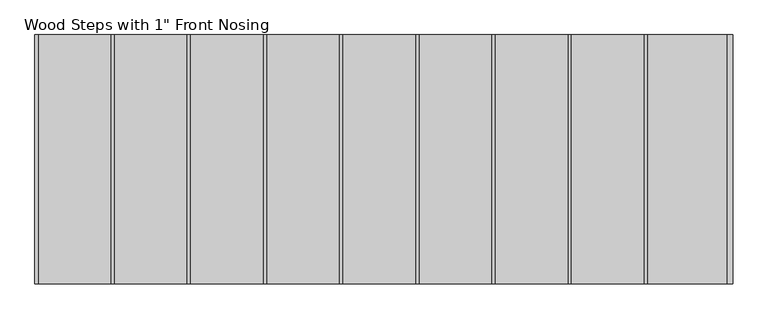
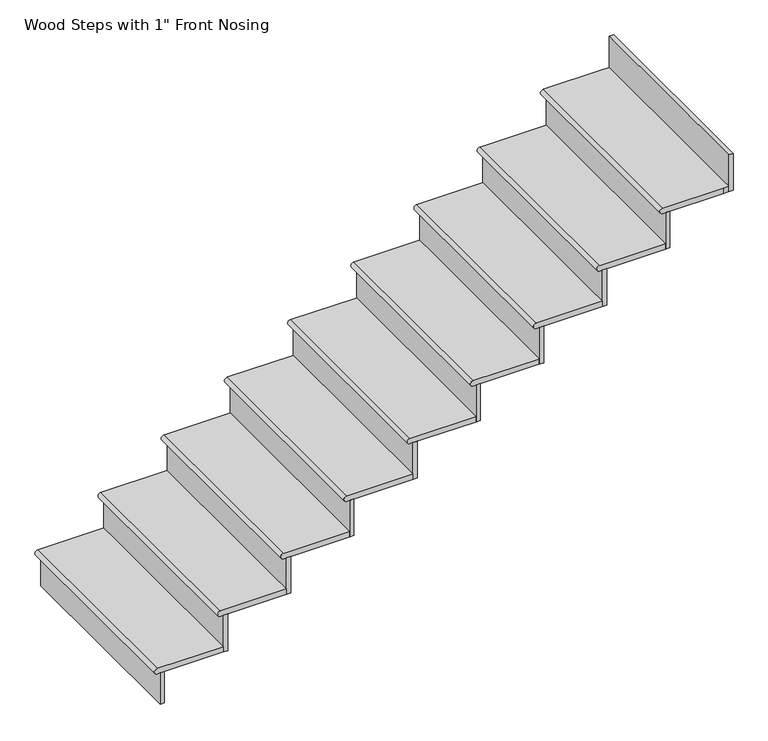
"""IFC4 building model written with IfcOpenShell, lengths in millimetres: stair flight geometry."""

import ifcopenshell
import ifcopenshell.guid

model = None  # the IFC model being written
_history = None  # IfcOwnerHistory: only IFC2X3 demands one
_inside = {}  # id of a spatial element -> (the spatial element, [elements in it])
_under = {}  # id of a project, library or spatial element -> (it, [spatial elements below it])
_declared = {}  # id of a project -> (the project, [libraries it declares])
_typed = {}  # id of a type object -> (the type object, [elements of that type])
_made_of = {}  # id of a material, layer set ... -> (it, [elements and type objects made of it])


def new_model(schema):
    """Start an empty IFC model of exactly this schema.

    Asked for "IFC4X3", IfcOpenShell would pick the latest addendum, in which some entities
    have other attributes; the version numbers below select the first issue.
    IFC2X3 requires an IfcOwnerHistory on every rooted entity: one is made here for all.
    """
    global model, _history
    if schema == "IFC4X3":
        model = ifcopenshell.file(schema_version=(4, 3, 0, 0))
    else:
        model = ifcopenshell.file(schema=schema)
    _inside.clear()
    _under.clear()
    _declared.clear()
    _typed.clear()
    _made_of.clear()
    _history = None
    if model.schema == "IFC2X3":
        org = make("IfcOrganization", Name="unknown")
        user = make(
            "IfcPersonAndOrganization",
            ThePerson=make("IfcPerson", FamilyName="unknown"),
            TheOrganization=org,
        )
        app = make(
            "IfcApplication",
            ApplicationDeveloper=org,
            Version="unknown",
            ApplicationFullName="unknown",
            ApplicationIdentifier="unknown",
        )
        _history = make(
            "IfcOwnerHistory",
            OwningUser=user,
            OwningApplication=app,
            ChangeAction="ADDED",
            CreationDate=0,
        )
    return model


def make(cls, **values):
    """One entity of the class cls with the attributes given. An attribute that is None is left unset."""
    return model.create_entity(
        cls, **{name: value for name, value in values.items() if value is not None}
    )


def rooted(cls, **values):
    """An entity with a GlobalId (a new one), such as an element, a storey or a relation."""
    return make(cls, GlobalId=ifcopenshell.guid.new(), OwnerHistory=_history, **values)


def si_unit(unit_type, name, prefix=None):
    """IfcSIUnit, for example si_unit("LENGTHUNIT", "METRE", prefix="MILLI")."""
    return make("IfcSIUnit", UnitType=unit_type, Prefix=prefix, Name=name)


def assignment(units):
    """IfcUnitAssignment: the units of a project."""
    return None if units is None else make("IfcUnitAssignment", Units=units)


def point(xyz):
    """IfcCartesianPoint."""
    return None if xyz is None else make("IfcCartesianPoint", Coordinates=xyz)


def direction(xyz):
    """IfcDirection."""
    return None if xyz is None else make("IfcDirection", DirectionRatios=xyz)


def frame(location, z_axis=None, x_axis=None):
    """IfcAxis2Placement3D, a coordinate frame: its origin and axes. An axis left out is left unset."""
    return make(
        "IfcAxis2Placement3D",
        Location=point(location),
        Axis=direction(z_axis),
        RefDirection=direction(x_axis),
    )


def origin():
    """The frame at (0, 0, 0) with its axes left unset."""
    return frame((0.0, 0.0, 0.0))


def place(relative_to, where):
    """IfcLocalPlacement: puts the frame where relative to a parent placement (None: the world)."""
    return make(
        "IfcLocalPlacement", PlacementRelTo=relative_to, RelativePlacement=where
    )


def context(
    kind, dimensions, precision=None, world=None, true_north=None, identifier=None
):
    """IfcGeometricRepresentationContext, for example the 3D "Model" context."""
    return make(
        "IfcGeometricRepresentationContext",
        ContextIdentifier=identifier,
        ContextType=kind,
        CoordinateSpaceDimension=dimensions,
        Precision=precision,
        WorldCoordinateSystem=world,
        TrueNorth=true_north,
    )


def project(units=None, contexts=None):
    """IfcProject with its units and contexts."""
    return rooted(
        "IfcProject",
        Name="project",
        RepresentationContexts=contexts,
        UnitsInContext=assignment(units),
    )


def spatial(cls, under=None, at=None, **own):
    """A site, building, storey or space (cls), placed at a placement, below another one or the project."""
    s = rooted(cls, ObjectPlacement=at, **own)
    if under is not None:
        _under.setdefault(under.id(), (under, []))[1].append(s)
    return s


def circle_curve(where, radius):
    """IfcCircle in the frame where."""
    return make("IfcCircle", Position=where, Radius=radius)


def faces_of(points, faces, orient=None, outer=None):
    """IfcFace entities. A face is a list of loops; a loop is a list of indices into points, from 0.

    orient and outer hold one flag for each loop. By default every Orientation is true, the
    first loop of a face is its IfcFaceOuterBound and the others are IfcFaceBound.
    """
    made = []
    for i, loops in enumerate(faces):
        bounds = []
        for j, loop in enumerate(loops):
            is_outer = j == 0 if outer is None else outer[i][j]
            bounds.append(
                make(
                    "IfcFaceOuterBound" if is_outer else "IfcFaceBound",
                    Bound=make("IfcPolyLoop", Polygon=[points[k] for k in loop]),
                    Orientation=True if orient is None else orient[i][j],
                )
            )
        made.append(make("IfcFace", Bounds=bounds))
    return made


def faceted_brep(points, faces, orient=None, outer=None, voids=None):
    """IfcFacetedBrep: a solid bounded by flat faces; with voids (closed shells), ...WithVoids."""
    shared = [point(p) for p in points]
    hull = make("IfcClosedShell", CfsFaces=faces_of(shared, faces, orient, outer))
    if voids is None:
        return make("IfcFacetedBrep", Outer=hull)
    return make(
        "IfcFacetedBrepWithVoids",
        Outer=hull,
        Voids=[
            make(cls, CfsFaces=faces_of(shared, fs, o, b)) for cls, fs, o, b in voids
        ],
    )


def shape(context_of_items, identifier, shape_type, items):
    """IfcShapeRepresentation: the items that make up one representation, for example the "Body"."""
    return make(
        "IfcShapeRepresentation",
        ContextOfItems=context_of_items,
        RepresentationIdentifier=identifier,
        RepresentationType=shape_type,
        Items=items,
    )


def source(mapping_origin, context_of_items, identifier, shape_type, items):
    """IfcRepresentationMap: a shape defined once, which mapped items show again and again."""
    return make(
        "IfcRepresentationMap",
        MappingOrigin=mapping_origin,
        MappedRepresentation=shape(context_of_items, identifier, shape_type, items),
    )


def transform(
    local_origin,
    x_axis=None,
    y_axis=None,
    z_axis=None,
    scale=None,
    scale2=None,
    scale3=None,
    uniform=True,
):
    """IfcCartesianTransformationOperator3D, or its non-uniform kind. x_axis, y_axis, z_axis: its Axis1, 2, 3."""
    if uniform:
        return make(
            "IfcCartesianTransformationOperator3D",
            Axis1=direction(x_axis),
            Axis2=direction(y_axis),
            LocalOrigin=point(local_origin),
            Scale=scale,
            Axis3=direction(z_axis),
        )
    return make(
        "IfcCartesianTransformationOperator3DnonUniform",
        Axis1=direction(x_axis),
        Axis2=direction(y_axis),
        LocalOrigin=point(local_origin),
        Scale=scale,
        Axis3=direction(z_axis),
        Scale2=scale2,
        Scale3=scale3,
    )


def mapped(mapping_source, mapping_target):
    """IfcMappedItem: shows the shape of a source again, moved by a transform."""
    return make(
        "IfcMappedItem", MappingSource=mapping_source, MappingTarget=mapping_target
    )


def made_of(thing, what):
    """Note that an element or type object is made of a material, layer set ...; save() writes the relation."""
    if what is not None:
        _made_of.setdefault(what.id(), (what, []))[1].append(thing)
    return thing


def element(
    cls,
    number,
    at=None,
    inside=None,
    cuts=None,
    type_object=None,
    material=None,
    context=None,
    identifier="Body",
    shape_type=None,
    held_by="IfcProductDefinitionShape",
    body=None,
    shapes=None,
    **own,
):
    """One element of the class cls, such as IfcWall. Its Tag is "e" and its number.

    at: its placement. inside: the storey or other place that contains it. cuts: it is an
    opening in that element (IfcRelVoidsElement). A single representation is given by context,
    identifier, shape_type and body (its items); several are given by shapes. held_by: the class
    of the entity that holds the representations. save() writes the other relations.
    """
    e = rooted(cls, Tag="e%d" % number, ObjectPlacement=at, **own)
    if body is not None:
        shapes = [shape(context, identifier, shape_type, body)]
    if shapes is not None:
        e.Representation = make(held_by, Representations=shapes)
    if inside is not None:
        _inside.setdefault(inside.id(), (inside, []))[1].append(e)
    if cuts is not None:
        rooted(
            "IfcRelVoidsElement", RelatingBuildingElement=cuts, RelatedOpeningElement=e
        )
    if type_object is not None:
        _typed.setdefault(type_object.id(), (type_object, []))[1].append(e)
    return made_of(e, material)


def aggregate(whole, parts):
    """IfcRelAggregates: a whole, such as a stair, and the parts it consists of."""
    return rooted("IfcRelAggregates", RelatingObject=whole, RelatedObjects=parts)


def save(model, path):
    """Write the relations noted so far, then the file.

    IfcRelAggregates (storeys below a building ...), IfcRelContainedInSpatialStructure (elements
    in a storey), IfcRelDefinesByType, IfcRelAssociatesMaterial and IfcRelDeclares: one each for
    every whole, place, type object, material and project.
    """
    for whole, parts in _under.values():
        aggregate(whole, parts)
    for where, things in _inside.values():
        rooted(
            "IfcRelContainedInSpatialStructure",
            RelatedElements=things,
            RelatingStructure=where,
        )
    for kind, things in _typed.values():
        rooted("IfcRelDefinesByType", RelatedObjects=things, RelatingType=kind)
    for what, things in _made_of.values():
        rooted("IfcRelAssociatesMaterial", RelatedObjects=things, RelatingMaterial=what)
    for by, libraries in _declared.values():
        rooted("IfcRelDeclares", RelatingContext=by, RelatedDefinitions=libraries)
    model.write(path)


def plane_surface(at):
    """IfcPlane: the flat surface through the origin of the frame at, square to its z axis."""
    return make("IfcPlane", Position=at)


def cylinder_surface(at, radius):
    """IfcCylindricalSurface: all points at the distance radius from the z axis of the frame at."""
    return make("IfcCylindricalSurface", Position=at, Radius=radius)


def advanced_brep(points, edges, surfaces, faces):
    """IfcAdvancedBrep: a solid bounded by faces that lie on surfaces and meet in shared edges.

    An edge is (start, end): straight between two places in points (the first is 0);
    or (start, end, curve); or (start, end, curve, False) where it runs against its curve.
    A face is (place in surfaces, loops), or (place, loops, False) where it looks against
    its surface's normal. A loop lists edges by number (the first is 1), with a minus sign
    where the edge is run from its end to its start. The first loop is the outer one.
    """
    corners = [point(p) for p in points]
    vertices = [make("IfcVertexPoint", VertexGeometry=c) for c in corners]
    made = []
    for start, end, *more in edges:
        made.append(
            make(
                "IfcEdgeCurve",
                EdgeStart=vertices[start],
                EdgeEnd=vertices[end],
                EdgeGeometry=more[0] if more else make("IfcPolyline", Points=[corners[start], corners[end]]),
                SameSense=more[1] if len(more) > 1 else True,
            )
        )
    hull = []
    for where, loops, *sense in faces:
        bounds = []
        for j, loop in enumerate(loops):
            ring = [make("IfcOrientedEdge", EdgeElement=made[abs(k) - 1], Orientation=k > 0) for k in loop]
            bounds.append(
                make(
                    "IfcFaceOuterBound" if j == 0 else "IfcFaceBound",
                    Bound=make("IfcEdgeLoop", EdgeList=ring),
                    Orientation=True,
                )
            )
        hull.append(make("IfcAdvancedFace", Bounds=bounds, FaceSurface=surfaces[where], SameSense=sense[0] if sense else True))
    return make("IfcAdvancedBrep", Outer=make("IfcClosedShell", CfsFaces=hull))


def stair_flight_bb49cb81(model_context):
    return source(origin(), model_context, "Body", "SolidModel", [
        advanced_brep(
        [(3725.1741968, -13363.3557429, 146.05), (3725.1741968, -13363.3557429, 171.45), (3725.1741968, -12448.9557429, 171.45), (3725.1741968, -12448.9557429, 146.05), (4017.2741968, -12448.9557429, 171.45), (4017.2741968, -13363.3557429, 171.45), (4017.2741968, -12448.9557429, 146.05), (4017.2741968, -13363.3557429, 146.05)],
        [
            (0, 1, circle_curve(frame((3725.1741968, -13363.3557429, 158.75), z_axis=(0.0, 1.0, 0.0), x_axis=(1.0, 0.0, 0.0)), 12.7)),
            (1, 2),
            (2, 3, circle_curve(frame((3725.1741968, -12448.9557429, 158.75), z_axis=(0.0, -1.0, 0.0), x_axis=(1.0, 0.0, 0.0)), 12.7)),
            (3, 0),
            (4, 2),
            (1, 5),
            (5, 4),
            (3, 6),
            (6, 7),
            (7, 0),
            (4, 6),
            (7, 5),
        ],
        [
            cylinder_surface(frame((3725.1741968, -13363.3557429, 158.75), z_axis=(0.0, -1.0, 0.0), x_axis=(1.0, 0.0, 0.0)), 12.7),
            plane_surface(frame((3712.4741968, -12448.9557429, 171.45), z_axis=(0.0, 0.0, 1.0), x_axis=(-1.0, 0.0, 0.0))),
            plane_surface(frame((3712.4741968, -12448.9557429, 146.05), z_axis=(0.0, 0.0, -1.0), x_axis=(1.0, 0.0, 0.0))),
            plane_surface(frame((4017.2741968, -12448.9557429, 171.45), z_axis=(0.0, 1.0, 0.0), x_axis=(0.0, 0.0, -1.0))),
            plane_surface(frame((3725.1741968, -13363.3557429, 171.45), z_axis=(0.0, -1.0, 0.0), x_axis=(0.0, 0.0, -1.0))),
            plane_surface(frame((4017.2741968, -13363.3557429, 171.45), z_axis=(1.0, 0.0, 0.0), x_axis=(0.0, 0.0, -1.0))),
        ],
        [
            (0, [[1, 2, 3, 4]]),
            (1, [[5, -2, 6, 7]]),
            (2, [[8, 9, 10, -4]]),
            (3, [[-5, 11, -8, -3]]),
            (4, [[-6, -1, -10, 12]]),
            (5, [[-7, -12, -9, -11]]),
        ],
    ),
        faceted_brep([(3737.8741968, -13363.3557429, 146.05), (3737.8741968, -13363.3557429, 0.0), (3756.9241968, -13363.3557429, 0.0), (3756.9241968, -13363.3557429, 146.05), (3737.8741968, -12448.9557429, 146.05), (3756.9241968, -12448.9557429, 146.05), (3756.9241968, -12448.9557429, 0.0), (3737.8741968, -12448.9557429, 0.0)], [[[0, 1, 2, 3]], [[4, 5, 6, 7]], [[1, 0, 4, 7]], [[2, 1, 7, 6]], [[3, 2, 6, 5]], [[0, 3, 5, 4]]]),
        faceted_brep([(4017.2741968, -13363.3557429, 317.5), (4017.2741968, -13363.3557429, 146.05), (4036.3241968, -13363.3557429, 146.05), (4036.3241968, -13363.3557429, 317.5), (4017.2741968, -12448.9557429, 317.5), (4036.3241968, -12448.9557429, 317.5), (4036.3241968, -12448.9557429, 146.05), (4017.2741968, -12448.9557429, 146.05)], [[[0, 1, 2, 3]], [[4, 5, 6, 7]], [[1, 0, 4, 7]], [[2, 1, 7, 6]], [[3, 2, 6, 5]], [[0, 3, 5, 4]]]),
        advanced_brep(
        [(4296.6741968, -12448.9557429, 342.9), (4004.5741968, -12448.9557429, 342.9), (4004.5741968, -13363.3557429, 342.9), (4296.6741968, -13363.3557429, 342.9), (4004.5741968, -12448.9557429, 317.5), (4296.6741968, -12448.9557429, 317.5), (4296.6741968, -13363.3557429, 317.5), (4004.5741968, -13363.3557429, 317.5)],
        [
            (0, 1),
            (1, 2),
            (2, 3),
            (3, 0),
            (4, 5),
            (5, 6),
            (6, 7),
            (7, 4),
            (0, 5),
            (4, 1, circle_curve(frame((4004.5741968, -12448.9557429, 330.2), z_axis=(0.0, 1.0, 0.0), x_axis=(1.0, 0.0, 0.0)), 12.7)),
            (2, 7, circle_curve(frame((4004.5741968, -13363.3557429, 330.2), z_axis=(0.0, -1.0, 0.0), x_axis=(1.0, 0.0, 0.0)), 12.7)),
            (6, 3),
        ],
        [
            plane_surface(frame((3712.4741968, -12448.9557429, 342.9), z_axis=(0.0, 0.0, 1.0), x_axis=(-1.0, 0.0, 0.0))),
            plane_surface(frame((3712.4741968, -12448.9557429, 317.5), z_axis=(0.0, 0.0, -1.0), x_axis=(1.0, 0.0, 0.0))),
            plane_surface(frame((4296.6741968, -12448.9557429, 342.9), z_axis=(0.0, 1.0, 0.0), x_axis=(0.0, 0.0, -1.0))),
            plane_surface(frame((4004.5741968, -13363.3557429, 342.9), z_axis=(0.0, -1.0, 0.0), x_axis=(0.0, 0.0, -1.0))),
            plane_surface(frame((4296.6741968, -13363.3557429, 342.9), z_axis=(1.0, 0.0, 0.0), x_axis=(0.0, 0.0, -1.0))),
            cylinder_surface(frame((4004.5741968, -13363.3557429, 330.2), z_axis=(0.0, -1.0, 0.0), x_axis=(1.0, 0.0, 0.0)), 12.7),
        ],
        [
            (0, [[1, 2, 3, 4]]),
            (1, [[5, 6, 7, 8]]),
            (2, [[-1, 9, -5, 10]]),
            (3, [[-3, 11, -7, 12]]),
            (4, [[-4, -12, -6, -9]]),
            (5, [[-11, -2, -10, -8]]),
        ],
    ),
        faceted_brep([(4296.6741968, -13363.3557429, 488.95), (4296.6741968, -13363.3557429, 317.5), (4315.7241968, -13363.3557429, 317.5), (4315.7241968, -13363.3557429, 488.95), (4296.6741968, -12448.9557429, 488.95), (4315.7241968, -12448.9557429, 488.95), (4315.7241968, -12448.9557429, 317.5), (4296.6741968, -12448.9557429, 317.5)], [[[0, 1, 2, 3]], [[4, 5, 6, 7]], [[1, 0, 4, 7]], [[2, 1, 7, 6]], [[3, 2, 6, 5]], [[0, 3, 5, 4]]]),
        advanced_brep(
        [(4576.0741968, -12448.9557429, 514.35), (4283.9741968, -12448.9557429, 514.35), (4283.9741968, -13363.3557429, 514.35), (4576.0741968, -13363.3557429, 514.35), (4283.9741968, -12448.9557429, 488.95), (4576.0741968, -12448.9557429, 488.95), (4576.0741968, -13363.3557429, 488.95), (4283.9741968, -13363.3557429, 488.95)],
        [
            (0, 1),
            (1, 2),
            (2, 3),
            (3, 0),
            (4, 5),
            (5, 6),
            (6, 7),
            (7, 4),
            (0, 5),
            (4, 1, circle_curve(frame((4283.9741968, -12448.9557429, 501.65), z_axis=(0.0, 1.0, 0.0), x_axis=(1.0, 0.0, 0.0)), 12.7)),
            (2, 7, circle_curve(frame((4283.9741968, -13363.3557429, 501.65), z_axis=(0.0, -1.0, 0.0), x_axis=(1.0, 0.0, 0.0)), 12.7)),
            (6, 3),
        ],
        [
            plane_surface(frame((3991.8741968, -12448.9557429, 514.35), z_axis=(0.0, 0.0, 1.0), x_axis=(-1.0, 0.0, 0.0))),
            plane_surface(frame((3991.8741968, -12448.9557429, 488.95), z_axis=(0.0, 0.0, -1.0), x_axis=(1.0, 0.0, 0.0))),
            plane_surface(frame((4576.0741968, -12448.9557429, 514.35), z_axis=(0.0, 1.0, 0.0), x_axis=(0.0, 0.0, -1.0))),
            plane_surface(frame((4283.9741968, -13363.3557429, 514.35), z_axis=(0.0, -1.0, 0.0), x_axis=(0.0, 0.0, -1.0))),
            plane_surface(frame((4576.0741968, -13363.3557429, 514.35), z_axis=(1.0, 0.0, 0.0), x_axis=(0.0, 0.0, -1.0))),
            cylinder_surface(frame((4283.9741968, -13363.3557429, 501.65), z_axis=(0.0, -1.0, 0.0), x_axis=(1.0, 0.0, 0.0)), 12.7),
        ],
        [
            (0, [[1, 2, 3, 4]]),
            (1, [[5, 6, 7, 8]]),
            (2, [[-1, 9, -5, 10]]),
            (3, [[-3, 11, -7, 12]]),
            (4, [[-4, -12, -6, -9]]),
            (5, [[-11, -2, -10, -8]]),
        ],
    ),
        faceted_brep([(4576.0741968, -13363.3557429, 660.4), (4576.0741968, -13363.3557429, 488.95), (4595.1241968, -13363.3557429, 488.95), (4595.1241968, -13363.3557429, 660.4), (4576.0741968, -12448.9557429, 660.4), (4595.1241968, -12448.9557429, 660.4), (4595.1241968, -12448.9557429, 488.95), (4576.0741968, -12448.9557429, 488.95)], [[[0, 1, 2, 3]], [[4, 5, 6, 7]], [[1, 0, 4, 7]], [[2, 1, 7, 6]], [[3, 2, 6, 5]], [[0, 3, 5, 4]]]),
        advanced_brep(
        [(4855.4741968, -12448.9557429, 685.8), (4563.3741968, -12448.9557429, 685.8), (4563.3741968, -13363.3557429, 685.8), (4855.4741968, -13363.3557429, 685.8), (4563.3741968, -12448.9557429, 660.4), (4855.4741968, -12448.9557429, 660.4), (4855.4741968, -13363.3557429, 660.4), (4563.3741968, -13363.3557429, 660.4)],
        [
            (0, 1),
            (1, 2),
            (2, 3),
            (3, 0),
            (4, 5),
            (5, 6),
            (6, 7),
            (7, 4),
            (0, 5),
            (4, 1, circle_curve(frame((4563.3741968, -12448.9557429, 673.1), z_axis=(0.0, 1.0, 0.0), x_axis=(1.0, 0.0, 0.0)), 12.7)),
            (2, 7, circle_curve(frame((4563.3741968, -13363.3557429, 673.1), z_axis=(0.0, -1.0, 0.0), x_axis=(1.0, 0.0, 0.0)), 12.7)),
            (6, 3),
        ],
        [
            plane_surface(frame((4271.2741968, -12448.9557429, 685.8), z_axis=(0.0, 0.0, 1.0), x_axis=(-1.0, 0.0, 0.0))),
            plane_surface(frame((4271.2741968, -12448.9557429, 660.4), z_axis=(0.0, 0.0, -1.0), x_axis=(1.0, 0.0, 0.0))),
            plane_surface(frame((4855.4741968, -12448.9557429, 685.8), z_axis=(0.0, 1.0, 0.0), x_axis=(0.0, 0.0, -1.0))),
            plane_surface(frame((4563.3741968, -13363.3557429, 685.8), z_axis=(0.0, -1.0, 0.0), x_axis=(0.0, 0.0, -1.0))),
            plane_surface(frame((4855.4741968, -13363.3557429, 685.8), z_axis=(1.0, 0.0, 0.0), x_axis=(0.0, 0.0, -1.0))),
            cylinder_surface(frame((4563.3741968, -13363.3557429, 673.1), z_axis=(0.0, -1.0, 0.0), x_axis=(1.0, 0.0, 0.0)), 12.7),
        ],
        [
            (0, [[1, 2, 3, 4]]),
            (1, [[5, 6, 7, 8]]),
            (2, [[-1, 9, -5, 10]]),
            (3, [[-3, 11, -7, 12]]),
            (4, [[-4, -12, -6, -9]]),
            (5, [[-11, -2, -10, -8]]),
        ],
    ),
        faceted_brep([(4855.4741968, -13363.3557429, 831.85), (4855.4741968, -13363.3557429, 660.4), (4874.5241968, -13363.3557429, 660.4), (4874.5241968, -13363.3557429, 831.85), (4855.4741968, -12448.9557429, 831.85), (4874.5241968, -12448.9557429, 831.85), (4874.5241968, -12448.9557429, 660.4), (4855.4741968, -12448.9557429, 660.4)], [[[0, 1, 2, 3]], [[4, 5, 6, 7]], [[1, 0, 4, 7]], [[2, 1, 7, 6]], [[3, 2, 6, 5]], [[0, 3, 5, 4]]]),
        advanced_brep(
        [(5134.8741968, -12448.9557429, 857.25), (4842.7741968, -12448.9557429, 857.25), (4842.7741968, -13363.3557429, 857.25), (5134.8741968, -13363.3557429, 857.25), (4842.7741968, -12448.9557429, 831.85), (5134.8741968, -12448.9557429, 831.85), (5134.8741968, -13363.3557429, 831.85), (4842.7741968, -13363.3557429, 831.85)],
        [
            (0, 1),
            (1, 2),
            (2, 3),
            (3, 0),
            (4, 5),
            (5, 6),
            (6, 7),
            (7, 4),
            (0, 5),
            (4, 1, circle_curve(frame((4842.7741968, -12448.9557429, 844.55), z_axis=(0.0, 1.0, 0.0), x_axis=(1.0, 0.0, 0.0)), 12.7)),
            (2, 7, circle_curve(frame((4842.7741968, -13363.3557429, 844.55), z_axis=(0.0, -1.0, 0.0), x_axis=(1.0, 0.0, 0.0)), 12.7)),
            (6, 3),
        ],
        [
            plane_surface(frame((4550.6741968, -12448.9557429, 857.25), z_axis=(0.0, 0.0, 1.0), x_axis=(-1.0, 0.0, 0.0))),
            plane_surface(frame((4550.6741968, -12448.9557429, 831.85), z_axis=(0.0, 0.0, -1.0), x_axis=(1.0, 0.0, 0.0))),
            plane_surface(frame((5134.8741968, -12448.9557429, 857.25), z_axis=(0.0, 1.0, 0.0), x_axis=(0.0, 0.0, -1.0))),
            plane_surface(frame((4842.7741968, -13363.3557429, 857.25), z_axis=(0.0, -1.0, 0.0), x_axis=(0.0, 0.0, -1.0))),
            plane_surface(frame((5134.8741968, -13363.3557429, 857.25), z_axis=(1.0, 0.0, 0.0), x_axis=(0.0, 0.0, -1.0))),
            cylinder_surface(frame((4842.7741968, -13363.3557429, 844.55), z_axis=(0.0, -1.0, 0.0), x_axis=(1.0, 0.0, 0.0)), 12.7),
        ],
        [
            (0, [[1, 2, 3, 4]]),
            (1, [[5, 6, 7, 8]]),
            (2, [[-1, 9, -5, 10]]),
            (3, [[-3, 11, -7, 12]]),
            (4, [[-4, -12, -6, -9]]),
            (5, [[-11, -2, -10, -8]]),
        ],
    ),
        faceted_brep([(5134.8741968, -13363.3557429, 1003.3), (5134.8741968, -13363.3557429, 831.85), (5153.9241968, -13363.3557429, 831.85), (5153.9241968, -13363.3557429, 1003.3), (5134.8741968, -12448.9557429, 1003.3), (5153.9241968, -12448.9557429, 1003.3), (5153.9241968, -12448.9557429, 831.85), (5134.8741968, -12448.9557429, 831.85)], [[[0, 1, 2, 3]], [[4, 5, 6, 7]], [[1, 0, 4, 7]], [[2, 1, 7, 6]], [[3, 2, 6, 5]], [[0, 3, 5, 4]]]),
        advanced_brep(
        [(5414.2741968, -12448.9557429, 1028.7), (5122.1741968, -12448.9557429, 1028.7), (5122.1741968, -13363.3557429, 1028.7), (5414.2741968, -13363.3557429, 1028.7), (5122.1741968, -12448.9557429, 1003.3), (5414.2741968, -12448.9557429, 1003.3), (5414.2741968, -13363.3557429, 1003.3), (5122.1741968, -13363.3557429, 1003.3)],
        [
            (0, 1),
            (1, 2),
            (2, 3),
            (3, 0),
            (4, 5),
            (5, 6),
            (6, 7),
            (7, 4),
            (0, 5),
            (4, 1, circle_curve(frame((5122.1741968, -12448.9557429, 1016.0), z_axis=(0.0, 1.0, 0.0), x_axis=(1.0, 0.0, 0.0)), 12.7)),
            (2, 7, circle_curve(frame((5122.1741968, -13363.3557429, 1016.0), z_axis=(0.0, -1.0, 0.0), x_axis=(1.0, 0.0, 0.0)), 12.7)),
            (6, 3),
        ],
        [
            plane_surface(frame((4830.0741968, -12448.9557429, 1028.7), z_axis=(0.0, 0.0, 1.0), x_axis=(-1.0, 0.0, 0.0))),
            plane_surface(frame((4830.0741968, -12448.9557429, 1003.3), z_axis=(0.0, 0.0, -1.0), x_axis=(1.0, 0.0, 0.0))),
            plane_surface(frame((5414.2741968, -12448.9557429, 1028.7), z_axis=(0.0, 1.0, 0.0), x_axis=(0.0, 0.0, -1.0))),
            plane_surface(frame((5122.1741968, -13363.3557429, 1028.7), z_axis=(0.0, -1.0, 0.0), x_axis=(0.0, 0.0, -1.0))),
            plane_surface(frame((5414.2741968, -13363.3557429, 1028.7), z_axis=(1.0, 0.0, 0.0), x_axis=(0.0, 0.0, -1.0))),
            cylinder_surface(frame((5122.1741968, -13363.3557429, 1016.0), z_axis=(0.0, -1.0, 0.0), x_axis=(1.0, 0.0, 0.0)), 12.7),
        ],
        [
            (0, [[1, 2, 3, 4]]),
            (1, [[5, 6, 7, 8]]),
            (2, [[-1, 9, -5, 10]]),
            (3, [[-3, 11, -7, 12]]),
            (4, [[-4, -12, -6, -9]]),
            (5, [[-11, -2, -10, -8]]),
        ],
    ),
        faceted_brep([(5414.2741968, -13363.3557429, 1174.75), (5414.2741968, -13363.3557429, 1003.3), (5433.3241968, -13363.3557429, 1003.3), (5433.3241968, -13363.3557429, 1174.75), (5414.2741968, -12448.9557429, 1174.75), (5433.3241968, -12448.9557429, 1174.75), (5433.3241968, -12448.9557429, 1003.3), (5414.2741968, -12448.9557429, 1003.3)], [[[0, 1, 2, 3]], [[4, 5, 6, 7]], [[1, 0, 4, 7]], [[2, 1, 7, 6]], [[3, 2, 6, 5]], [[0, 3, 5, 4]]]),
        advanced_brep(
        [(5693.6741968, -12448.9557429, 1200.15), (5401.5741968, -12448.9557429, 1200.15), (5401.5741968, -13363.3557429, 1200.15), (5693.6741968, -13363.3557429, 1200.15), (5401.5741968, -12448.9557429, 1174.75), (5693.6741968, -12448.9557429, 1174.75), (5693.6741968, -13363.3557429, 1174.75), (5401.5741968, -13363.3557429, 1174.75)],
        [
            (0, 1),
            (1, 2),
            (2, 3),
            (3, 0),
            (4, 5),
            (5, 6),
            (6, 7),
            (7, 4),
            (0, 5),
            (4, 1, circle_curve(frame((5401.5741968, -12448.9557429, 1187.45), z_axis=(0.0, 1.0, 0.0), x_axis=(1.0, 0.0, 0.0)), 12.7)),
            (2, 7, circle_curve(frame((5401.5741968, -13363.3557429, 1187.45), z_axis=(0.0, -1.0, 0.0), x_axis=(1.0, 0.0, 0.0)), 12.7)),
            (6, 3),
        ],
        [
            plane_surface(frame((5109.4741968, -12448.9557429, 1200.15), z_axis=(0.0, 0.0, 1.0), x_axis=(-1.0, 0.0, 0.0))),
            plane_surface(frame((5109.4741968, -12448.9557429, 1174.75), z_axis=(0.0, 0.0, -1.0), x_axis=(1.0, 0.0, 0.0))),
            plane_surface(frame((5693.6741968, -12448.9557429, 1200.15), z_axis=(0.0, 1.0, 0.0), x_axis=(0.0, 0.0, -1.0))),
            plane_surface(frame((5401.5741968, -13363.3557429, 1200.15), z_axis=(0.0, -1.0, 0.0), x_axis=(0.0, 0.0, -1.0))),
            plane_surface(frame((5693.6741968, -13363.3557429, 1200.15), z_axis=(1.0, 0.0, 0.0), x_axis=(0.0, 0.0, -1.0))),
            cylinder_surface(frame((5401.5741968, -13363.3557429, 1187.45), z_axis=(0.0, -1.0, 0.0), x_axis=(1.0, 0.0, 0.0)), 12.7),
        ],
        [
            (0, [[1, 2, 3, 4]]),
            (1, [[5, 6, 7, 8]]),
            (2, [[-1, 9, -5, 10]]),
            (3, [[-3, 11, -7, 12]]),
            (4, [[-4, -12, -6, -9]]),
            (5, [[-11, -2, -10, -8]]),
        ],
    ),
        faceted_brep([(5693.6741968, -13363.3557429, 1346.2), (5693.6741968, -13363.3557429, 1174.75), (5712.7241968, -13363.3557429, 1174.75), (5712.7241968, -13363.3557429, 1346.2), (5693.6741968, -12448.9557429, 1346.2), (5712.7241968, -12448.9557429, 1346.2), (5712.7241968, -12448.9557429, 1174.75), (5693.6741968, -12448.9557429, 1174.75)], [[[0, 1, 2, 3]], [[4, 5, 6, 7]], [[1, 0, 4, 7]], [[2, 1, 7, 6]], [[3, 2, 6, 5]], [[0, 3, 5, 4]]]),
        advanced_brep(
        [(5973.0741968, -12448.9557429, 1371.6), (5680.9741968, -12448.9557429, 1371.6), (5680.9741968, -13363.3557429, 1371.6), (5973.0741968, -13363.3557429, 1371.6), (5680.9741968, -12448.9557429, 1346.2), (5973.0741968, -12448.9557429, 1346.2), (5973.0741968, -13363.3557429, 1346.2), (5680.9741968, -13363.3557429, 1346.2)],
        [
            (0, 1),
            (1, 2),
            (2, 3),
            (3, 0),
            (4, 5),
            (5, 6),
            (6, 7),
            (7, 4),
            (0, 5),
            (4, 1, circle_curve(frame((5680.9741968, -12448.9557429, 1358.9), z_axis=(0.0, 1.0, 0.0), x_axis=(1.0, 0.0, 0.0)), 12.7)),
            (2, 7, circle_curve(frame((5680.9741968, -13363.3557429, 1358.9), z_axis=(0.0, -1.0, 0.0), x_axis=(1.0, 0.0, 0.0)), 12.7)),
            (6, 3),
        ],
        [
            plane_surface(frame((5388.8741968, -12448.9557429, 1371.6), z_axis=(0.0, 0.0, 1.0), x_axis=(-1.0, 0.0, 0.0))),
            plane_surface(frame((5388.8741968, -12448.9557429, 1346.2), z_axis=(0.0, 0.0, -1.0), x_axis=(1.0, 0.0, 0.0))),
            plane_surface(frame((5973.0741968, -12448.9557429, 1371.6), z_axis=(0.0, 1.0, 0.0), x_axis=(0.0, 0.0, -1.0))),
            plane_surface(frame((5680.9741968, -13363.3557429, 1371.6), z_axis=(0.0, -1.0, 0.0), x_axis=(0.0, 0.0, -1.0))),
            plane_surface(frame((5973.0741968, -13363.3557429, 1371.6), z_axis=(1.0, 0.0, 0.0), x_axis=(0.0, 0.0, -1.0))),
            cylinder_surface(frame((5680.9741968, -13363.3557429, 1358.9), z_axis=(0.0, -1.0, 0.0), x_axis=(1.0, 0.0, 0.0)), 12.7),
        ],
        [
            (0, [[1, 2, 3, 4]]),
            (1, [[5, 6, 7, 8]]),
            (2, [[-1, 9, -5, 10]]),
            (3, [[-3, 11, -7, 12]]),
            (4, [[-4, -12, -6, -9]]),
            (5, [[-11, -2, -10, -8]]),
        ],
    ),
        faceted_brep([(6252.4741968, -13363.3557429, 1689.1), (6252.4741968, -13363.3557429, 1517.65), (6271.5241968, -13363.3557429, 1517.65), (6271.5241968, -13363.3557429, 1689.1), (6252.4741968, -12448.9557429, 1689.1), (6271.5241968, -12448.9557429, 1689.1), (6271.5241968, -12448.9557429, 1517.65), (6252.4741968, -12448.9557429, 1517.65)], [[[0, 1, 2, 3]], [[4, 5, 6, 7]], [[1, 0, 4, 7]], [[2, 1, 7, 6]], [[3, 2, 6, 5]], [[0, 3, 5, 4]]]),
        faceted_brep([(5973.0741968, -13363.3557429, 1517.65), (5973.0741968, -13363.3557429, 1346.2), (5992.1241968, -13363.3557429, 1346.2), (5992.1241968, -13363.3557429, 1517.65), (5973.0741968, -12448.9557429, 1517.65), (5992.1241968, -12448.9557429, 1517.65), (5992.1241968, -12448.9557429, 1346.2), (5973.0741968, -12448.9557429, 1346.2)], [[[0, 1, 2, 3]], [[4, 5, 6, 7]], [[1, 0, 4, 7]], [[2, 1, 7, 6]], [[3, 2, 6, 5]], [[0, 3, 5, 4]]]),
        advanced_brep(
        [(6252.4741968, -12448.9557429, 1543.05), (6227.0741968, -12448.9557429, 1543.05), (5960.3741968, -12448.9557429, 1543.05), (5960.3741968, -13363.3557429, 1543.05), (6227.0741968, -13363.3557429, 1543.05), (6252.4741968, -13363.3557429, 1543.05), (6227.0741968, -12448.9557429, 1517.65), (6252.4741968, -12448.9557429, 1517.65), (6252.4741968, -13363.3557429, 1517.65), (6227.0741968, -13363.3557429, 1517.65), (5960.3741968, -13363.3557429, 1517.65), (5960.3741968, -12448.9557429, 1517.65)],
        [
            (0, 1),
            (1, 2),
            (2, 3),
            (3, 4),
            (4, 5),
            (5, 0),
            (6, 7),
            (7, 8),
            (8, 9),
            (9, 10),
            (10, 11),
            (11, 6),
            (0, 7),
            (6, 1),
            (11, 2, circle_curve(frame((5960.3741968, -12448.9557429, 1530.35), z_axis=(0.0, 1.0, 0.0), x_axis=(1.0, 0.0, 0.0)), 12.7)),
            (3, 10, circle_curve(frame((5960.3741968, -13363.3557429, 1530.35), z_axis=(0.0, -1.0, 0.0), x_axis=(1.0, 0.0, 0.0)), 12.7)),
            (9, 4),
            (8, 5),
        ],
        [
            plane_surface(frame((6227.0741968, -12448.9557429, 1543.05), z_axis=(0.0, 0.0, 1.0), x_axis=(-1.0, 0.0, 0.0))),
            plane_surface(frame((6227.0741968, -12448.9557429, 1517.65), z_axis=(0.0, 0.0, -1.0), x_axis=(1.0, 0.0, 0.0))),
            plane_surface(frame((6252.4741968, -12448.9557429, 1543.05), z_axis=(0.0, 1.0, 0.0), x_axis=(0.0, 0.0, -1.0))),
            plane_surface(frame((6227.0741968, -12448.9557429, 1543.05), z_axis=(0.0, 1.0, 0.0), x_axis=(0.0, 0.0, -1.0))),
            plane_surface(frame((5960.3741968, -13363.3557429, 1543.05), z_axis=(0.0, -1.0, 0.0), x_axis=(0.0, 0.0, -1.0))),
            plane_surface(frame((6227.0741968, -13363.3557429, 1543.05), z_axis=(0.0, -1.0, 0.0), x_axis=(0.0, 0.0, -1.0))),
            plane_surface(frame((6252.4741968, -13363.3557429, 1543.05), z_axis=(1.0, 0.0, 0.0), x_axis=(0.0, 0.0, -1.0))),
            cylinder_surface(frame((5960.3741968, -13363.3557429, 1530.35), z_axis=(0.0, -1.0, 0.0), x_axis=(1.0, 0.0, 0.0)), 12.7),
        ],
        [
            (0, [[1, 2, 3, 4, 5, 6]]),
            (1, [[7, 8, 9, 10, 11, 12]]),
            (2, [[-1, 13, -7, 14]]),
            (3, [[-2, -14, -12, 15]]),
            (4, [[-4, 16, -10, 17]]),
            (5, [[-5, -17, -9, 18]]),
            (6, [[-6, -18, -8, -13]]),
            (7, [[-16, -3, -15, -11]]),
        ],
    ),
    ])


if __name__ == "__main__":
    model = new_model("IFC4")
    model_context = context("Model", 3, world=origin())
    ifc_project = project(units=[si_unit("LENGTHUNIT", "METRE", prefix="MILLI")], contexts=[model_context])
    site = spatial("IfcSite", under=ifc_project)
    building = spatial("IfcBuilding", under=site)
    placement = place(None, origin())
    stair_flight_shape = stair_flight_bb49cb81(model_context)
    element("IfcStairFlight", 1, ObjectType="Wood Steps with 1\" Front Nosing", at=placement, inside=building, context=model_context, shape_type="MappedRepresentation", body=[
        mapped(stair_flight_shape, transform((0.0, 0.0, 0.0), x_axis=(1.0, 0.0, 0.0), y_axis=(0.0, 1.0, 0.0), z_axis=(0.0, 0.0, 1.0))),
    ])
    save(model, "model.ifc")

# Revit data of these elements
# Element 1 (IfcStairFlight, "Wood Steps with 1\" Front Nosing")
#   Materials on its faces: "Paints and Coatings", "Cherry"
# Materials
#   "Paints and Coatings": class "Paint", colour RGB 244 244 244, transparency 0, Description = "Interior finish", Cost = 0
#   "Cherry": class "Wood", colour RGB 233 182 144, transparency 0, Description = "Prunus Serotina", Cost = 0
